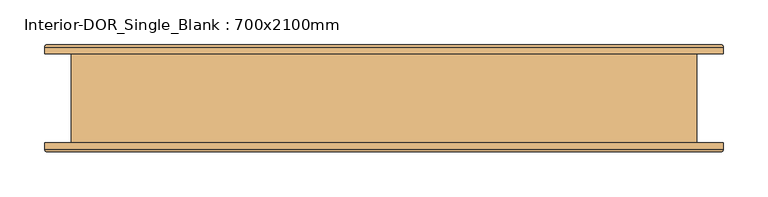
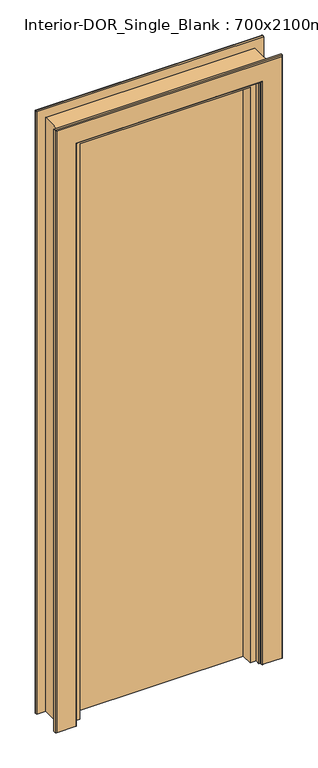
"""IFC4 building model written with IfcOpenShell, lengths in millimetres: door geometry, Interior-DOR_Single_Blank : 700x2100mm."""

import ifcopenshell
import ifcopenshell.guid

model = None  # the IFC model being written
_history = None  # IfcOwnerHistory: only IFC2X3 demands one
_inside = {}  # id of a spatial element -> (the spatial element, [elements in it])
_under = {}  # id of a project, library or spatial element -> (it, [spatial elements below it])
_declared = {}  # id of a project -> (the project, [libraries it declares])
_typed = {}  # id of a type object -> (the type object, [elements of that type])
_made_of = {}  # id of a material, layer set ... -> (it, [elements and type objects made of it])


def new_model(schema):
    """Start an empty IFC model of exactly this schema.

    Asked for "IFC4X3", IfcOpenShell would pick the latest addendum, in which some entities
    have other attributes; the version numbers below select the first issue.
    IFC2X3 requires an IfcOwnerHistory on every rooted entity: one is made here for all.
    """
    global model, _history
    if schema == "IFC4X3":
        model = ifcopenshell.file(schema_version=(4, 3, 0, 0))
    else:
        model = ifcopenshell.file(schema=schema)
    _inside.clear()
    _under.clear()
    _declared.clear()
    _typed.clear()
    _made_of.clear()
    _history = None
    if model.schema == "IFC2X3":
        org = make("IfcOrganization", Name="unknown")
        user = make(
            "IfcPersonAndOrganization",
            ThePerson=make("IfcPerson", FamilyName="unknown"),
            TheOrganization=org,
        )
        app = make(
            "IfcApplication",
            ApplicationDeveloper=org,
            Version="unknown",
            ApplicationFullName="unknown",
            ApplicationIdentifier="unknown",
        )
        _history = make(
            "IfcOwnerHistory",
            OwningUser=user,
            OwningApplication=app,
            ChangeAction="ADDED",
            CreationDate=0,
        )
    return model


def make(cls, **values):
    """One entity of the class cls with the attributes given. An attribute that is None is left unset."""
    return model.create_entity(
        cls, **{name: value for name, value in values.items() if value is not None}
    )


def rooted(cls, **values):
    """An entity with a GlobalId (a new one), such as an element, a storey or a relation."""
    return make(cls, GlobalId=ifcopenshell.guid.new(), OwnerHistory=_history, **values)


def si_unit(unit_type, name, prefix=None):
    """IfcSIUnit, for example si_unit("LENGTHUNIT", "METRE", prefix="MILLI")."""
    return make("IfcSIUnit", UnitType=unit_type, Prefix=prefix, Name=name)


def assignment(units):
    """IfcUnitAssignment: the units of a project."""
    return None if units is None else make("IfcUnitAssignment", Units=units)


def point(xyz):
    """IfcCartesianPoint."""
    return None if xyz is None else make("IfcCartesianPoint", Coordinates=xyz)


def direction(xyz):
    """IfcDirection."""
    return None if xyz is None else make("IfcDirection", DirectionRatios=xyz)


def frame(location, z_axis=None, x_axis=None):
    """IfcAxis2Placement3D, a coordinate frame: its origin and axes. An axis left out is left unset."""
    return make(
        "IfcAxis2Placement3D",
        Location=point(location),
        Axis=direction(z_axis),
        RefDirection=direction(x_axis),
    )


def origin():
    """The frame at (0, 0, 0) with its axes left unset."""
    return frame((0.0, 0.0, 0.0))


def origin_with_axes():
    """The frame at (0, 0, 0) with the z axis (0, 0, 1) and the x axis (1, 0, 0) written out."""
    return frame((0.0, 0.0, 0.0), z_axis=(0.0, 0.0, 1.0), x_axis=(1.0, 0.0, 0.0))


def place(relative_to, where):
    """IfcLocalPlacement: puts the frame where relative to a parent placement (None: the world)."""
    return make(
        "IfcLocalPlacement", PlacementRelTo=relative_to, RelativePlacement=where
    )


def context(
    kind, dimensions, precision=None, world=None, true_north=None, identifier=None
):
    """IfcGeometricRepresentationContext, for example the 3D "Model" context."""
    return make(
        "IfcGeometricRepresentationContext",
        ContextIdentifier=identifier,
        ContextType=kind,
        CoordinateSpaceDimension=dimensions,
        Precision=precision,
        WorldCoordinateSystem=world,
        TrueNorth=true_north,
    )


def project(units=None, contexts=None):
    """IfcProject with its units and contexts."""
    return rooted(
        "IfcProject",
        Name="project",
        RepresentationContexts=contexts,
        UnitsInContext=assignment(units),
    )


def spatial(cls, under=None, at=None, **own):
    """A site, building, storey or space (cls), placed at a placement, below another one or the project."""
    s = rooted(cls, ObjectPlacement=at, **own)
    if under is not None:
        _under.setdefault(under.id(), (under, []))[1].append(s)
    return s


def polyline(points):
    """IfcPolyline through the points."""
    return make("IfcPolyline", Points=[point(p) for p in points])


def circle_curve(where, radius):
    """IfcCircle in the frame where."""
    return make("IfcCircle", Position=where, Radius=radius)


def ellipse_curve(where, semi_axis1, semi_axis2):
    """IfcEllipse in the frame where."""
    return make(
        "IfcEllipse", Position=where, SemiAxis1=semi_axis1, SemiAxis2=semi_axis2
    )


def outline(outer, holes=None, kind="AREA"):
    """IfcArbitraryClosedProfileDef: a profile drawn as a closed curve; with holes, ...WithVoids."""
    if holes is None:
        return make("IfcArbitraryClosedProfileDef", ProfileType=kind, OuterCurve=outer)
    return make(
        "IfcArbitraryProfileDefWithVoids",
        ProfileType=kind,
        OuterCurve=outer,
        InnerCurves=holes,
    )


def extrude(swept, where, along, depth):
    """IfcExtrudedAreaSolid: the profile swept, set in the frame where, extruded along a direction by depth."""
    return make(
        "IfcExtrudedAreaSolid",
        SweptArea=swept,
        Position=where,
        ExtrudedDirection=direction(along),
        Depth=depth,
    )


def faces_of(points, faces, orient=None, outer=None):
    """IfcFace entities. A face is a list of loops; a loop is a list of indices into points, from 0.

    orient and outer hold one flag for each loop. By default every Orientation is true, the
    first loop of a face is its IfcFaceOuterBound and the others are IfcFaceBound.
    """
    made = []
    for i, loops in enumerate(faces):
        bounds = []
        for j, loop in enumerate(loops):
            is_outer = j == 0 if outer is None else outer[i][j]
            bounds.append(
                make(
                    "IfcFaceOuterBound" if is_outer else "IfcFaceBound",
                    Bound=make("IfcPolyLoop", Polygon=[points[k] for k in loop]),
                    Orientation=True if orient is None else orient[i][j],
                )
            )
        made.append(make("IfcFace", Bounds=bounds))
    return made


def faceted_brep(points, faces, orient=None, outer=None, voids=None):
    """IfcFacetedBrep: a solid bounded by flat faces; with voids (closed shells), ...WithVoids."""
    shared = [point(p) for p in points]
    hull = make("IfcClosedShell", CfsFaces=faces_of(shared, faces, orient, outer))
    if voids is None:
        return make("IfcFacetedBrep", Outer=hull)
    return make(
        "IfcFacetedBrepWithVoids",
        Outer=hull,
        Voids=[
            make(cls, CfsFaces=faces_of(shared, fs, o, b)) for cls, fs, o, b in voids
        ],
    )


def shape(context_of_items, identifier, shape_type, items):
    """IfcShapeRepresentation: the items that make up one representation, for example the "Body"."""
    return make(
        "IfcShapeRepresentation",
        ContextOfItems=context_of_items,
        RepresentationIdentifier=identifier,
        RepresentationType=shape_type,
        Items=items,
    )


def source(mapping_origin, context_of_items, identifier, shape_type, items):
    """IfcRepresentationMap: a shape defined once, which mapped items show again and again."""
    return make(
        "IfcRepresentationMap",
        MappingOrigin=mapping_origin,
        MappedRepresentation=shape(context_of_items, identifier, shape_type, items),
    )


def transform(
    local_origin,
    x_axis=None,
    y_axis=None,
    z_axis=None,
    scale=None,
    scale2=None,
    scale3=None,
    uniform=True,
):
    """IfcCartesianTransformationOperator3D, or its non-uniform kind. x_axis, y_axis, z_axis: its Axis1, 2, 3."""
    if uniform:
        return make(
            "IfcCartesianTransformationOperator3D",
            Axis1=direction(x_axis),
            Axis2=direction(y_axis),
            LocalOrigin=point(local_origin),
            Scale=scale,
            Axis3=direction(z_axis),
        )
    return make(
        "IfcCartesianTransformationOperator3DnonUniform",
        Axis1=direction(x_axis),
        Axis2=direction(y_axis),
        LocalOrigin=point(local_origin),
        Scale=scale,
        Axis3=direction(z_axis),
        Scale2=scale2,
        Scale3=scale3,
    )


def mapped(mapping_source, mapping_target):
    """IfcMappedItem: shows the shape of a source again, moved by a transform."""
    return make(
        "IfcMappedItem", MappingSource=mapping_source, MappingTarget=mapping_target
    )


def made_of(thing, what):
    """Note that an element or type object is made of a material, layer set ...; save() writes the relation."""
    if what is not None:
        _made_of.setdefault(what.id(), (what, []))[1].append(thing)
    return thing


def element(
    cls,
    number,
    at=None,
    inside=None,
    cuts=None,
    type_object=None,
    material=None,
    context=None,
    identifier="Body",
    shape_type=None,
    held_by="IfcProductDefinitionShape",
    body=None,
    shapes=None,
    **own,
):
    """One element of the class cls, such as IfcWall. Its Tag is "e" and its number.

    at: its placement. inside: the storey or other place that contains it. cuts: it is an
    opening in that element (IfcRelVoidsElement). A single representation is given by context,
    identifier, shape_type and body (its items); several are given by shapes. held_by: the class
    of the entity that holds the representations. save() writes the other relations.
    """
    e = rooted(cls, Tag="e%d" % number, ObjectPlacement=at, **own)
    if body is not None:
        shapes = [shape(context, identifier, shape_type, body)]
    if shapes is not None:
        e.Representation = make(held_by, Representations=shapes)
    if inside is not None:
        _inside.setdefault(inside.id(), (inside, []))[1].append(e)
    if cuts is not None:
        rooted(
            "IfcRelVoidsElement", RelatingBuildingElement=cuts, RelatedOpeningElement=e
        )
    if type_object is not None:
        _typed.setdefault(type_object.id(), (type_object, []))[1].append(e)
    return made_of(e, material)


def aggregate(whole, parts):
    """IfcRelAggregates: a whole, such as a stair, and the parts it consists of."""
    return rooted("IfcRelAggregates", RelatingObject=whole, RelatedObjects=parts)


def save(model, path):
    """Write the relations noted so far, then the file.

    IfcRelAggregates (storeys below a building ...), IfcRelContainedInSpatialStructure (elements
    in a storey), IfcRelDefinesByType, IfcRelAssociatesMaterial and IfcRelDeclares: one each for
    every whole, place, type object, material and project.
    """
    for whole, parts in _under.values():
        aggregate(whole, parts)
    for where, things in _inside.values():
        rooted(
            "IfcRelContainedInSpatialStructure",
            RelatedElements=things,
            RelatingStructure=where,
        )
    for kind, things in _typed.values():
        rooted("IfcRelDefinesByType", RelatedObjects=things, RelatingType=kind)
    for what, things in _made_of.values():
        rooted("IfcRelAssociatesMaterial", RelatedObjects=things, RelatingMaterial=what)
    for by, libraries in _declared.values():
        rooted("IfcRelDeclares", RelatingContext=by, RelatedDefinitions=libraries)
    model.write(path)


def plane_surface(at):
    """IfcPlane: the flat surface through the origin of the frame at, square to its z axis."""
    return make("IfcPlane", Position=at)


def cylinder_surface(at, radius):
    """IfcCylindricalSurface: all points at the distance radius from the z axis of the frame at."""
    return make("IfcCylindricalSurface", Position=at, Radius=radius)


def advanced_brep(points, edges, surfaces, faces):
    """IfcAdvancedBrep: a solid bounded by faces that lie on surfaces and meet in shared edges.

    An edge is (start, end): straight between two places in points (the first is 0);
    or (start, end, curve); or (start, end, curve, False) where it runs against its curve.
    A face is (place in surfaces, loops), or (place, loops, False) where it looks against
    its surface's normal. A loop lists edges by number (the first is 1), with a minus sign
    where the edge is run from its end to its start. The first loop is the outer one.
    """
    corners = [point(p) for p in points]
    vertices = [make("IfcVertexPoint", VertexGeometry=c) for c in corners]
    made = []
    for start, end, *more in edges:
        made.append(
            make(
                "IfcEdgeCurve",
                EdgeStart=vertices[start],
                EdgeEnd=vertices[end],
                EdgeGeometry=more[0] if more else make("IfcPolyline", Points=[corners[start], corners[end]]),
                SameSense=more[1] if len(more) > 1 else True,
            )
        )
    hull = []
    for where, loops, *sense in faces:
        bounds = []
        for j, loop in enumerate(loops):
            ring = [make("IfcOrientedEdge", EdgeElement=made[abs(k) - 1], Orientation=k > 0) for k in loop]
            bounds.append(
                make(
                    "IfcFaceOuterBound" if j == 0 else "IfcFaceBound",
                    Bound=make("IfcEdgeLoop", EdgeList=ring),
                    Orientation=True,
                )
            )
        hull.append(make("IfcAdvancedFace", Bounds=bounds, FaceSurface=surfaces[where], SameSense=sense[0] if sense else True))
    return make("IfcAdvancedBrep", Outer=make("IfcClosedShell", CfsFaces=hull))


def interior_dor_single_blank_700x2100mm_59f542ac(model_context):
    return source(origin(), model_context, "Body", "SolidModel", [
        advanced_brep(
        [(-310.0, 50.0, 0.0), (-380.0, 50.0, 0.0), (-380.0, 57.0, 0.0), (-377.0, 60.0, 0.0), (-313.0, 60.0, 0.0), (-310.0, 57.0, 0.0), (-310.0, 57.0, 2060.0), (-310.0, 50.0, 2060.0), (-313.0, 60.0, 2063.0), (-377.0, 60.0, 2127.0), (377.0, 60.0, 2127.0), (377.0, 60.0, 0.0), (313.0, 60.0, 0.0), (313.0, 60.0, 2063.0), (-380.0, 57.0, 2130.0), (-380.0, 50.0, 2130.0), (310.0, 50.0, 2060.0), (310.0, 50.0, 0.0), (380.0, 50.0, 0.0), (380.0, 50.0, 2130.0), (310.0, 57.0, 0.0), (310.0, 57.0, 2060.0), (380.0, 57.0, 0.0), (380.0, 57.0, 2130.0)],
        [
            (0, 1),
            (1, 2),
            (2, 3, circle_curve(frame((-377.0, 57.0, 0.0), z_axis=(0.0, 0.0, -1.0), x_axis=(-1.0, 0.0, 0.0)), 3.0)),
            (3, 4),
            (4, 5, circle_curve(frame((-313.0, 57.0, 0.0), z_axis=(0.0, 0.0, -1.0), x_axis=(-1.0, 0.0, 0.0)), 3.0)),
            (5, 0),
            (5, 6),
            (6, 7),
            (7, 0),
            (4, 8),
            (8, 6, ellipse_curve(frame((-313.0, 57.0, 2063.0), z_axis=(-0.7071067811865475, 0.0, -0.7071067811865475), x_axis=(0.7071067811865474, 0.0, -0.7071067811865476)), 4.2426407, 3.0)),
            (3, 9),
            (9, 10),
            (10, 11),
            (11, 12),
            (12, 13),
            (13, 8),
            (2, 14),
            (14, 9, ellipse_curve(frame((-377.0, 57.0, 2127.0), z_axis=(-0.7071067811865475, 0.0, -0.7071067811865475), x_axis=(0.7071067811865474, 0.0, -0.7071067811865476)), 4.2426407, 3.0)),
            (1, 15),
            (15, 14),
            (7, 16),
            (16, 17),
            (17, 18),
            (18, 19),
            (19, 15),
            (12, 20, circle_curve(frame((313.0, 57.0, 0.0), z_axis=(0.0, 0.0, 1.0), x_axis=(1.0, 0.0, 0.0)), 3.0)),
            (20, 21),
            (21, 13, ellipse_curve(frame((313.0, 57.0, 2063.0), z_axis=(0.7071067811865475, 0.0, -0.7071067811865475), x_axis=(0.7071067811865474, 0.0, 0.7071067811865476)), 4.2426407, 3.0)),
            (17, 20),
            (11, 22, circle_curve(frame((377.0, 57.0, 0.0), z_axis=(0.0, 0.0, -1.0), x_axis=(1.0, 0.0, 0.0)), 3.0)),
            (22, 18),
            (23, 22),
            (10, 23, ellipse_curve(frame((377.0, 57.0, 2127.0), z_axis=(0.7071067811865475, 0.0, -0.7071067811865475), x_axis=(0.7071067811865474, 0.0, 0.7071067811865476)), 4.2426407, 3.0)),
            (23, 19),
            (16, 21),
            (6, 21),
            (14, 23),
        ],
        [
            plane_surface(frame((-350.0, -50.0, 0.0), z_axis=(0.0, 0.0, -1.0), x_axis=(0.0, 1.0, 0.0))),
            plane_surface(frame((-310.0, 50.0, 0.0), z_axis=(1.0, 0.0, 0.0), x_axis=(0.0, 0.0, 1.0))),
            cylinder_surface(frame((-313.0, 57.0, 0.0), z_axis=(0.0, 0.0, -1.0), x_axis=(-1.0, 0.0, 0.0)), 3.0),
            plane_surface(frame((-313.0, 60.0, 0.0), z_axis=(0.0, 1.0, 0.0), x_axis=(0.0, 0.0, 1.0))),
            cylinder_surface(frame((-377.0, 57.0, 0.0), z_axis=(0.0, 0.0, -1.0), x_axis=(-1.0, 0.0, 0.0)), 3.0),
            plane_surface(frame((-380.0, 57.0, 0.0), z_axis=(-1.0, 0.0, 0.0), x_axis=(0.0, 0.0, 1.0))),
            plane_surface(frame((-380.0, 50.0, 0.0), z_axis=(0.0, -1.0, 0.0), x_axis=(0.0, 0.0, 1.0))),
            cylinder_surface(frame((313.0, 57.0, 2100.0), z_axis=(0.0, 0.0, 1.0), x_axis=(1.0, 0.0, 0.0)), 3.0),
            plane_surface(frame((350.0, -50.0, 0.0), z_axis=(0.0, 0.0, -1.0), x_axis=(0.0, 1.0, 0.0))),
            cylinder_surface(frame((377.0, 57.0, 2100.0), z_axis=(0.0, 0.0, 1.0), x_axis=(1.0, 0.0, 0.0)), 3.0),
            plane_surface(frame((380.0, 57.0, 2130.0), z_axis=(1.0, 0.0, 0.0), x_axis=(0.0, 0.0, -1.0))),
            plane_surface(frame((310.0, 50.0, 2060.0), z_axis=(-1.0, 0.0, 0.0), x_axis=(0.0, 0.0, -1.0))),
            plane_surface(frame((-310.0, 50.0, 2060.0), z_axis=(0.0, 0.0, -1.0), x_axis=(1.0, 0.0, 0.0))),
            cylinder_surface(frame((-350.0, 57.0, 2063.0), z_axis=(-1.0, 0.0, 0.0), x_axis=(0.0, 0.0, 1.0)), 3.0),
            cylinder_surface(frame((-350.0, 57.0, 2127.0), z_axis=(-1.0, 0.0, 0.0), x_axis=(0.0, 0.0, 1.0)), 3.0),
            plane_surface(frame((-380.0, 57.0, 2130.0), z_axis=(0.0, 0.0, 1.0), x_axis=(1.0, 0.0, 0.0))),
        ],
        [
            (0, [[1, 2, 3, 4, 5, 6]]),
            (1, [[7, 8, 9, -6]]),
            (2, [[10, 11, -7, -5]]),
            (3, [[12, 13, 14, 15, 16, 17, -10, -4]]),
            (4, [[18, 19, -12, -3]]),
            (5, [[20, 21, -18, -2]]),
            (6, [[-9, 22, 23, 24, 25, 26, -20, -1]]),
            (7, [[-16, 27, 28, 29]]),
            (8, [[30, -27, -15, 31, 32, -24]]),
            (9, [[33, -31, -14, 34]]),
            (10, [[-25, -32, -33, 35]]),
            (11, [[-28, -30, -23, 36]]),
            (12, [[37, -36, -22, -8]]),
            (13, [[-17, -29, -37, -11]]),
            (14, [[38, -34, -13, -19]]),
            (15, [[-26, -35, -38, -21]]),
        ],
    ),
        advanced_brep(
        [(-380.0, -50.0, 0.0), (-310.0, -50.0, 0.0), (-310.0, -57.0, 0.0), (-313.0, -60.0, 0.0), (-377.0, -60.0, 0.0), (-380.0, -57.0, 0.0), (-380.0, -57.0, 2130.0), (-380.0, -50.0, 2130.0), (-377.0, -60.0, 2127.0), (-313.0, -60.0, 2063.0), (313.0, -60.0, 2063.0), (313.0, -60.0, 0.0), (377.0, -60.0, 0.0), (377.0, -60.0, 2127.0), (-310.0, -57.0, 2060.0), (-310.0, -50.0, 2060.0), (380.0, -50.0, 2130.0), (380.0, -50.0, 0.0), (310.0, -50.0, 0.0), (310.0, -50.0, 2060.0), (380.0, -57.0, 0.0), (380.0, -57.0, 2130.0), (310.0, -57.0, 0.0), (310.0, -57.0, 2060.0)],
        [
            (0, 1),
            (1, 2),
            (2, 3, circle_curve(frame((-313.0, -57.0, 0.0), z_axis=(0.0, 0.0, -1.0), x_axis=(-1.0, 0.0, 0.0)), 3.0)),
            (3, 4),
            (4, 5, circle_curve(frame((-377.0, -57.0, 0.0), z_axis=(0.0, 0.0, -1.0), x_axis=(-1.0, 0.0, 0.0)), 3.0)),
            (5, 0),
            (5, 6),
            (6, 7),
            (7, 0),
            (4, 8),
            (8, 6, ellipse_curve(frame((-377.0, -57.0, 2127.0), z_axis=(-0.7071067811865475, 0.0, -0.7071067811865475), x_axis=(0.7071067811865474, 0.0, -0.7071067811865476)), 4.2426407, 3.0)),
            (3, 9),
            (9, 10),
            (10, 11),
            (11, 12),
            (12, 13),
            (13, 8),
            (2, 14),
            (14, 9, ellipse_curve(frame((-313.0, -57.0, 2063.0), z_axis=(-0.7071067811865475, 0.0, -0.7071067811865475), x_axis=(0.7071067811865474, 0.0, -0.7071067811865476)), 4.2426407, 3.0)),
            (1, 15),
            (15, 14),
            (7, 16),
            (16, 17),
            (17, 18),
            (18, 19),
            (19, 15),
            (12, 20, circle_curve(frame((377.0, -57.0, 0.0), z_axis=(0.0, 0.0, 1.0), x_axis=(1.0, 0.0, 0.0)), 3.0)),
            (20, 21),
            (21, 13, ellipse_curve(frame((377.0, -57.0, 2127.0), z_axis=(0.7071067811865475, 0.0, -0.7071067811865475), x_axis=(0.7071067811865474, 0.0, 0.7071067811865476)), 4.2426407, 3.0)),
            (17, 20),
            (11, 22, circle_curve(frame((313.0, -57.0, 0.0), z_axis=(0.0, 0.0, -1.0), x_axis=(1.0, 0.0, 0.0)), 3.0)),
            (22, 18),
            (23, 22),
            (10, 23, ellipse_curve(frame((313.0, -57.0, 2063.0), z_axis=(0.7071067811865475, 0.0, -0.7071067811865475), x_axis=(0.7071067811865474, 0.0, 0.7071067811865476)), 4.2426407, 3.0)),
            (23, 19),
            (16, 21),
            (6, 21),
            (14, 23),
        ],
        [
            plane_surface(frame((-350.0, -50.0, 0.0), z_axis=(0.0, 0.0, -1.0), x_axis=(0.0, 1.0, 0.0))),
            plane_surface(frame((-380.0, -50.0, 0.0), z_axis=(-1.0, 0.0, 0.0), x_axis=(0.0, 0.0, 1.0))),
            cylinder_surface(frame((-377.0, -57.0, 0.0), z_axis=(0.0, 0.0, -1.0), x_axis=(-1.0, 0.0, 0.0)), 3.0),
            plane_surface(frame((-377.0, -60.0, 0.0), z_axis=(0.0, -1.0, 0.0), x_axis=(0.0, 0.0, 1.0))),
            cylinder_surface(frame((-313.0, -57.0, 0.0), z_axis=(0.0, 0.0, -1.0), x_axis=(-1.0, 0.0, 0.0)), 3.0),
            plane_surface(frame((-310.0, -57.0, 0.0), z_axis=(1.0, 0.0, 0.0), x_axis=(0.0, 0.0, 1.0))),
            plane_surface(frame((-310.0, -50.0, 0.0), z_axis=(0.0, 1.0, 0.0), x_axis=(0.0, 0.0, 1.0))),
            cylinder_surface(frame((377.0, -57.0, 2100.0), z_axis=(0.0, 0.0, 1.0), x_axis=(1.0, 0.0, 0.0)), 3.0),
            plane_surface(frame((350.0, -50.0, 0.0), z_axis=(0.0, 0.0, -1.0), x_axis=(0.0, 1.0, 0.0))),
            cylinder_surface(frame((313.0, -57.0, 2100.0), z_axis=(0.0, 0.0, 1.0), x_axis=(1.0, 0.0, 0.0)), 3.0),
            plane_surface(frame((310.0, -57.0, 2060.0), z_axis=(-1.0, 0.0, 0.0), x_axis=(0.0, 0.0, -1.0))),
            plane_surface(frame((380.0, -50.0, 2130.0), z_axis=(1.0, 0.0, 0.0), x_axis=(0.0, 0.0, -1.0))),
            plane_surface(frame((-380.0, -50.0, 2130.0), z_axis=(0.0, 0.0, 1.0), x_axis=(1.0, 0.0, 0.0))),
            cylinder_surface(frame((-350.0, -57.0, 2127.0), z_axis=(-1.0, 0.0, 0.0), x_axis=(0.0, 0.0, 1.0)), 3.0),
            cylinder_surface(frame((-350.0, -57.0, 2063.0), z_axis=(-1.0, 0.0, 0.0), x_axis=(0.0, 0.0, 1.0)), 3.0),
            plane_surface(frame((-310.0, -57.0, 2060.0), z_axis=(0.0, 0.0, -1.0), x_axis=(1.0, 0.0, 0.0))),
        ],
        [
            (0, [[1, 2, 3, 4, 5, 6]]),
            (1, [[7, 8, 9, -6]]),
            (2, [[10, 11, -7, -5]]),
            (3, [[12, 13, 14, 15, 16, 17, -10, -4]]),
            (4, [[18, 19, -12, -3]]),
            (5, [[20, 21, -18, -2]]),
            (6, [[-9, 22, 23, 24, 25, 26, -20, -1]]),
            (7, [[-16, 27, 28, 29]]),
            (8, [[30, -27, -15, 31, 32, -24]]),
            (9, [[33, -31, -14, 34]]),
            (10, [[-25, -32, -33, 35]]),
            (11, [[-28, -30, -23, 36]]),
            (12, [[37, -36, -22, -8]]),
            (13, [[-17, -29, -37, -11]]),
            (14, [[38, -34, -13, -19]]),
            (15, [[-26, -35, -38, -21]]),
        ],
    ),
        faceted_brep([(-350.0, -50.0, 0.0), (-350.0, 50.0, 0.0), (-305.0, 50.0, 0.0), (-305.0, 5.0, 0.0), (-285.0, 5.0, 0.0), (-285.0, -35.0, 0.0), (-305.0, -35.0, 0.0), (-305.0, -50.0, 0.0), (-305.0, -50.0, 2055.0), (305.0, -50.0, 2055.0), (305.0, -50.0, 0.0), (350.0, -50.0, 0.0), (350.0, -50.0, 2100.0), (-350.0, -50.0, 2100.0), (-305.0, -35.0, 2055.0), (-285.0, -35.0, 2035.0), (285.0, -35.0, 2035.0), (285.0, -35.0, 0.0), (305.0, -35.0, 0.0), (305.0, -35.0, 2055.0), (-285.0, 5.0, 2035.0), (-305.0, 5.0, 2055.0), (305.0, 5.0, 2055.0), (305.0, 5.0, 0.0), (285.0, 5.0, 0.0), (285.0, 5.0, 2035.0), (-305.0, 50.0, 2055.0), (-350.0, 50.0, 2100.0), (350.0, 50.0, 2100.0), (350.0, 50.0, 0.0), (305.0, 50.0, 0.0), (305.0, 50.0, 2055.0)], [[[0, 1, 2, 3, 4, 5, 6, 7]], [[7, 8, 9, 10, 11, 12, 13, 0]], [[6, 14, 8, 7]], [[5, 15, 16, 17, 18, 19, 14, 6]], [[4, 20, 15, 5]], [[3, 21, 22, 23, 24, 25, 20, 4]], [[2, 26, 21, 3]], [[1, 27, 28, 29, 30, 31, 26, 2]], [[0, 13, 27, 1]], [[12, 11, 29, 28]], [[11, 10, 18, 17, 24, 23, 30, 29]], [[19, 18, 10, 9]], [[25, 24, 17, 16]], [[31, 30, 23, 22]], [[20, 25, 16, 15]], [[26, 31, 22, 21]], [[13, 12, 28, 27]], [[14, 19, 9, 8]]]),
        extrude(outline(polyline([(305.0, 50.0), (305.0, 5.0), (-305.0, 5.0), (-305.0, 50.0), (305.0, 50.0)])), origin_with_axes(), (0.0, 0.0, 1.0), 2055.0),
    ])


if __name__ == "__main__":
    model = new_model("IFC4")
    model_context = context("Model", 3, world=origin())
    ifc_project = project(units=[si_unit("LENGTHUNIT", "METRE", prefix="MILLI")], contexts=[model_context])
    site = spatial("IfcSite", under=ifc_project)
    building = spatial("IfcBuilding", under=site)
    placement = place(None, origin())
    interior_dor_single_blank_700x2100mm_shape = interior_dor_single_blank_700x2100mm_59f542ac(model_context)
    element("IfcDoor", 1, ObjectType="Interior-DOR_Single_Blank : 700x2100mm", at=placement, inside=building, context=model_context, shape_type="MappedRepresentation", body=[
        mapped(interior_dor_single_blank_700x2100mm_shape, transform((0.0, 0.0, 0.0), x_axis=(1.0, 0.0, 0.0), y_axis=(0.0, 1.0, 0.0), z_axis=(0.0, 0.0, 1.0))),
    ])
    save(model, "model.ifc")

# Revit data of these elements
# Type "Interior-DOR_Single_Blank : 700x2100mm"
#   Type IfcGUID = "1sWU2cMPP4xwRoAc3TXQKN"
#   Assembly Code = "C1020120"
#   Type Mark = "196"
#   Classification.Uniclass.EF.Number = "EF_25_30"
#   Classification.Uniclass.EF.Description = "Doors and windows"
#   WindLoadRating = "n/a"
#   WaterTightnessRating = "n/a"
#   WarrantyStartDate [instance default] = "1900-12-31T23:59:59"
#   WarrantyGuarantorParts = "n/a"
#   WarrantyGuarantorLabor = "n/a"
#   WarrantyDurationUnit = "year"
#   WarrantyDurationParts = "n/a"
#   WarrantyDurationLabor = "n/a"
#   WarrantyDescription = "n/a"
#   Version = "2"
#   Uniclass2015Version = "Systems v1.9"
#   Uniclass2015Title = "Doorset systems"
#   Uniclass2015Code = "Ss_25_30_20_25"
#   URL = "www.nationalbimlibrary.com"
#   TagNumber [instance default] = "n/a"
#   SustainabilityPerformance = "n/a"
#   Status = "UNSET"
#   Size = "1010 x 2100 mm"
#   Shape = "n/a"
#   SerialNumber [instance default] = "n/a"
#   SecurityRating = "n/a"
#   Revision = "n/a"
#   ReplacementCost = "n/a"
#   Reference = "n/a"
#   ProductInformation = "n/a"
#   Operation = "SINGLE_SWING_RIGHT"
#   OmniClassVersion = "Table 22 2012-05-16"
#   OmniClassTitle = "Doors and Frames"
#   OmniClassCode = "22-08 10 00"
#   Name = "DoorsetSystem_Interior-Single_Blank"
#   NBSReference = "25-50-20/120"
#   NBSDescription = "Doorset system"
#   NBSCertification = "www.nationalbimlibrary.com/cert/mlf45nxc"
#   ModelReference = "Interior Single Door"
#   ModelNumber = "n/a"
#   Model = "Interior Single Door"
#   MechanicalLoadRating = "n/a"
#   Material = "n/a"
#   ManufacturerURL = "n/a"
#   ManufacturerName = "n/a"
#   Manufacturer = "info@theNBS.com"
#   InstallationDate [instance default] = "1900-12-31T23:59:59"
#   IfcExportType = "DOOR"
#   IfcExportAs = "IfcDoorType"
#   HygrothermalRating = "n/a"
#   Grade = "n/a"
#   FireRating = "n/a"
#   Fire Rating = "n/a"
#   Finish = "n/a"
#   Features = "n/a"
#   ExpectedLife = "n/a"
#   DurationUnit = "n/a"
#   DurabilityRating = "n/a"
#   DoorNumber [instance default] = "n/a"
#   Description = "Generic single interior door"
#   Construction Type = "USERDEFINED"
#   Constituents = "n/a"
#   ComponentNumber [instance default] = "n/a"
#   Color = "n/a"
#   CodePerformance = "n/a"
#   Category = "Ss_25_30_20_25:Doorset systems"
#   BarCode [instance default] = "n/a"
#   BIMObjectName = "NBS_DoorsetSystem_Interior-Single_Blank"
#   Author = "NBS"
#   AssetType = "Fixed"
#   AssetIdentifier [instance default] = "n/a"
#   AcousticRating = "n/a"
#   AccessibilityPerformance = "n/a"
#   Width = 0.7 m
#   WallThickness [instance default] = 0.15 m
#   ThresholdHeight = 0.015 m
#   Thickness = 0.15 m
#   ThermalTransmittance = 0
#   StructuralToleranceJamb = 0 m
#   StructuralToleranceHead = 0 m
#   StructuralOpeningWidth = 0.7 m
#   StructuralOpeningHeight = 2.1 m
#   StopProjection = 0.02 m
#   StopDepth = 0.04 m
#   Rough Width [instance default] = 0.7 m
#   Rough Height [instance default] = 2.1 m
#   RebateDepth = 0.045 m
#   PanelWidth = 0.61 m
#   PanelUndercut = 0 m
#   PanelHeight = 2.055 m
#   PanelDepth = 0.045 m
#   OpeningTolerance = 0 m
#   NominalWidth = 0.7 m
#   NominalLength = 0 m
#   NominalHeight = 2.1 m
#   Infiltration = 0
#   Height = 2.1 m
#   GlazingAreaFraction = 0
#   FrameThickness = 0.045 m
#   FrameSetback [instance default] = 0 m
#   FrameDepth [instance default] = 0.15 m
#   FinishThicknessInternal [instance default] = 0 m
#   FinishThicknessExternal [instance default] = 0 m
#   ClearOpeningWidth = 0.57 m
#   ClearOpeningHeight = 2.035 m
#   CalculatedInteriorVoidDepth [instance default] = 0.3 m
#   ArchitraveWidth = 0.07 m
#   ArchitraveThickness = 0.01 m
#   ArchitraveSetbackFromFrameFace = 0.005 m
#   SmokeStop = no
#   SingleRebate = no
#   SelfClosing = no
#   PlantedStop = yes
#   IsExternal = no
#   HasDrive = no
#   HandicapAccessible = no
#   Wall Closure = 4
#   FireExit = no
#   ArchitraveFrontRequired [instance default] = yes
#   ArchitraveBackRequired [instance default] = yes
#   PanelMaterial = NBS_Concept
#   HardwareFinish = NBS_Concept
#   FrameSectionMaterial = NBS_Concept
#   Function = (empty or 0)
#   Cost = 0
# Element 1 (IfcDoor, "Interior-DOR_Single_Blank : 700x2100mm")
#   WallThickness = 0.1 m
#   FrameDepth = 0.1 m
#   Materials on its faces: "NBS_Concept"
# Materials
#   "NBS_Concept": class "Generic", colour RGB 255 255 255, transparency 0, Description = "To be specified", Cost = 0
